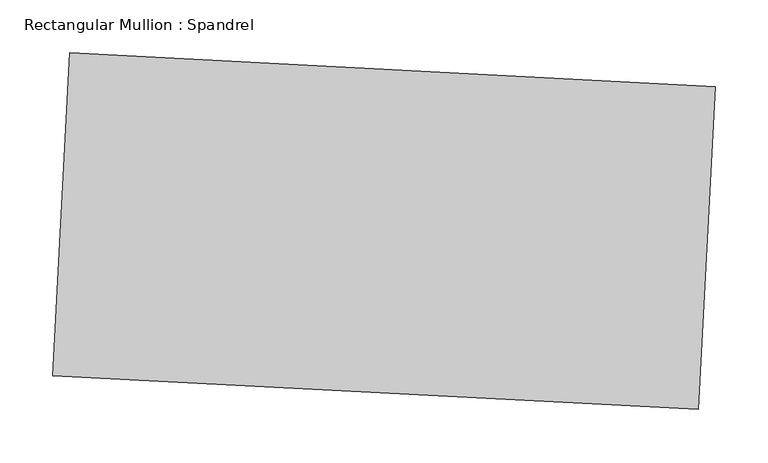
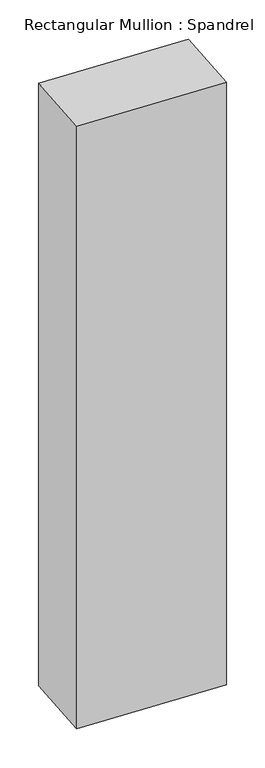
"""IFC4 building model written with IfcOpenShell, lengths in millimetres: member geometry, Rectangular Mullion : Spandrel."""

import ifcopenshell
import ifcopenshell.guid

model = None  # the IFC model being written
_history = None  # IfcOwnerHistory: only IFC2X3 demands one
_inside = {}  # id of a spatial element -> (the spatial element, [elements in it])
_under = {}  # id of a project, library or spatial element -> (it, [spatial elements below it])
_declared = {}  # id of a project -> (the project, [libraries it declares])
_typed = {}  # id of a type object -> (the type object, [elements of that type])
_made_of = {}  # id of a material, layer set ... -> (it, [elements and type objects made of it])


def new_model(schema):
    """Start an empty IFC model of exactly this schema.

    Asked for "IFC4X3", IfcOpenShell would pick the latest addendum, in which some entities
    have other attributes; the version numbers below select the first issue.
    IFC2X3 requires an IfcOwnerHistory on every rooted entity: one is made here for all.
    """
    global model, _history
    if schema == "IFC4X3":
        model = ifcopenshell.file(schema_version=(4, 3, 0, 0))
    else:
        model = ifcopenshell.file(schema=schema)
    _inside.clear()
    _under.clear()
    _declared.clear()
    _typed.clear()
    _made_of.clear()
    _history = None
    if model.schema == "IFC2X3":
        org = make("IfcOrganization", Name="unknown")
        user = make(
            "IfcPersonAndOrganization",
            ThePerson=make("IfcPerson", FamilyName="unknown"),
            TheOrganization=org,
        )
        app = make(
            "IfcApplication",
            ApplicationDeveloper=org,
            Version="unknown",
            ApplicationFullName="unknown",
            ApplicationIdentifier="unknown",
        )
        _history = make(
            "IfcOwnerHistory",
            OwningUser=user,
            OwningApplication=app,
            ChangeAction="ADDED",
            CreationDate=0,
        )
    return model


def make(cls, **values):
    """One entity of the class cls with the attributes given. An attribute that is None is left unset."""
    return model.create_entity(
        cls, **{name: value for name, value in values.items() if value is not None}
    )


def rooted(cls, **values):
    """An entity with a GlobalId (a new one), such as an element, a storey or a relation."""
    return make(cls, GlobalId=ifcopenshell.guid.new(), OwnerHistory=_history, **values)


def si_unit(unit_type, name, prefix=None):
    """IfcSIUnit, for example si_unit("LENGTHUNIT", "METRE", prefix="MILLI")."""
    return make("IfcSIUnit", UnitType=unit_type, Prefix=prefix, Name=name)


def assignment(units):
    """IfcUnitAssignment: the units of a project."""
    return None if units is None else make("IfcUnitAssignment", Units=units)


def point(xyz):
    """IfcCartesianPoint."""
    return None if xyz is None else make("IfcCartesianPoint", Coordinates=xyz)


def direction(xyz):
    """IfcDirection."""
    return None if xyz is None else make("IfcDirection", DirectionRatios=xyz)


def frame(location, z_axis=None, x_axis=None):
    """IfcAxis2Placement3D, a coordinate frame: its origin and axes. An axis left out is left unset."""
    return make(
        "IfcAxis2Placement3D",
        Location=point(location),
        Axis=direction(z_axis),
        RefDirection=direction(x_axis),
    )


def origin():
    """The frame at (0, 0, 0) with its axes left unset."""
    return frame((0.0, 0.0, 0.0))


def place(relative_to, where):
    """IfcLocalPlacement: puts the frame where relative to a parent placement (None: the world)."""
    return make(
        "IfcLocalPlacement", PlacementRelTo=relative_to, RelativePlacement=where
    )


def context(
    kind, dimensions, precision=None, world=None, true_north=None, identifier=None
):
    """IfcGeometricRepresentationContext, for example the 3D "Model" context."""
    return make(
        "IfcGeometricRepresentationContext",
        ContextIdentifier=identifier,
        ContextType=kind,
        CoordinateSpaceDimension=dimensions,
        Precision=precision,
        WorldCoordinateSystem=world,
        TrueNorth=true_north,
    )


def project(units=None, contexts=None):
    """IfcProject with its units and contexts."""
    return rooted(
        "IfcProject",
        Name="project",
        RepresentationContexts=contexts,
        UnitsInContext=assignment(units),
    )


def spatial(cls, under=None, at=None, **own):
    """A site, building, storey or space (cls), placed at a placement, below another one or the project."""
    s = rooted(cls, ObjectPlacement=at, **own)
    if under is not None:
        _under.setdefault(under.id(), (under, []))[1].append(s)
    return s


def polyline(points):
    """IfcPolyline through the points."""
    return make("IfcPolyline", Points=[point(p) for p in points])


def outline(outer, holes=None, kind="AREA"):
    """IfcArbitraryClosedProfileDef: a profile drawn as a closed curve; with holes, ...WithVoids."""
    if holes is None:
        return make("IfcArbitraryClosedProfileDef", ProfileType=kind, OuterCurve=outer)
    return make(
        "IfcArbitraryProfileDefWithVoids",
        ProfileType=kind,
        OuterCurve=outer,
        InnerCurves=holes,
    )


def extrude(swept, where, along, depth):
    """IfcExtrudedAreaSolid: the profile swept, set in the frame where, extruded along a direction by depth."""
    return make(
        "IfcExtrudedAreaSolid",
        SweptArea=swept,
        Position=where,
        ExtrudedDirection=direction(along),
        Depth=depth,
    )


def shape(context_of_items, identifier, shape_type, items):
    """IfcShapeRepresentation: the items that make up one representation, for example the "Body"."""
    return make(
        "IfcShapeRepresentation",
        ContextOfItems=context_of_items,
        RepresentationIdentifier=identifier,
        RepresentationType=shape_type,
        Items=items,
    )


def source(mapping_origin, context_of_items, identifier, shape_type, items):
    """IfcRepresentationMap: a shape defined once, which mapped items show again and again."""
    return make(
        "IfcRepresentationMap",
        MappingOrigin=mapping_origin,
        MappedRepresentation=shape(context_of_items, identifier, shape_type, items),
    )


def transform(
    local_origin,
    x_axis=None,
    y_axis=None,
    z_axis=None,
    scale=None,
    scale2=None,
    scale3=None,
    uniform=True,
):
    """IfcCartesianTransformationOperator3D, or its non-uniform kind. x_axis, y_axis, z_axis: its Axis1, 2, 3."""
    if uniform:
        return make(
            "IfcCartesianTransformationOperator3D",
            Axis1=direction(x_axis),
            Axis2=direction(y_axis),
            LocalOrigin=point(local_origin),
            Scale=scale,
            Axis3=direction(z_axis),
        )
    return make(
        "IfcCartesianTransformationOperator3DnonUniform",
        Axis1=direction(x_axis),
        Axis2=direction(y_axis),
        LocalOrigin=point(local_origin),
        Scale=scale,
        Axis3=direction(z_axis),
        Scale2=scale2,
        Scale3=scale3,
    )


def mapped(mapping_source, mapping_target):
    """IfcMappedItem: shows the shape of a source again, moved by a transform."""
    return make(
        "IfcMappedItem", MappingSource=mapping_source, MappingTarget=mapping_target
    )


def made_of(thing, what):
    """Note that an element or type object is made of a material, layer set ...; save() writes the relation."""
    if what is not None:
        _made_of.setdefault(what.id(), (what, []))[1].append(thing)
    return thing


def element(
    cls,
    number,
    at=None,
    inside=None,
    cuts=None,
    type_object=None,
    material=None,
    context=None,
    identifier="Body",
    shape_type=None,
    held_by="IfcProductDefinitionShape",
    body=None,
    shapes=None,
    **own,
):
    """One element of the class cls, such as IfcWall. Its Tag is "e" and its number.

    at: its placement. inside: the storey or other place that contains it. cuts: it is an
    opening in that element (IfcRelVoidsElement). A single representation is given by context,
    identifier, shape_type and body (its items); several are given by shapes. held_by: the class
    of the entity that holds the representations. save() writes the other relations.
    """
    e = rooted(cls, Tag="e%d" % number, ObjectPlacement=at, **own)
    if body is not None:
        shapes = [shape(context, identifier, shape_type, body)]
    if shapes is not None:
        e.Representation = make(held_by, Representations=shapes)
    if inside is not None:
        _inside.setdefault(inside.id(), (inside, []))[1].append(e)
    if cuts is not None:
        rooted(
            "IfcRelVoidsElement", RelatingBuildingElement=cuts, RelatedOpeningElement=e
        )
    if type_object is not None:
        _typed.setdefault(type_object.id(), (type_object, []))[1].append(e)
    return made_of(e, material)


def aggregate(whole, parts):
    """IfcRelAggregates: a whole, such as a stair, and the parts it consists of."""
    return rooted("IfcRelAggregates", RelatingObject=whole, RelatedObjects=parts)


def save(model, path):
    """Write the relations noted so far, then the file.

    IfcRelAggregates (storeys below a building ...), IfcRelContainedInSpatialStructure (elements
    in a storey), IfcRelDefinesByType, IfcRelAssociatesMaterial and IfcRelDeclares: one each for
    every whole, place, type object, material and project.
    """
    for whole, parts in _under.values():
        aggregate(whole, parts)
    for where, things in _inside.values():
        rooted(
            "IfcRelContainedInSpatialStructure",
            RelatedElements=things,
            RelatingStructure=where,
        )
    for kind, things in _typed.values():
        rooted("IfcRelDefinesByType", RelatedObjects=things, RelatingType=kind)
    for what, things in _made_of.values():
        rooted("IfcRelAssociatesMaterial", RelatedObjects=things, RelatingMaterial=what)
    for by, libraries in _declared.values():
        rooted("IfcRelDeclares", RelatingContext=by, RelatedDefinitions=libraries)
    model.write(path)


def rectangular_mullion_spandrel_2df0ba9b(model_context):
    return source(origin(), model_context, "Body", "SweptSolid", [
        extrude(outline(polyline([(312.3582819, 136.2391416), (296.4062825, -168.1431406), (-312.3582819, -136.2391416), (-296.4062825, 168.1431406), (312.3582819, 136.2391416)])), frame((0.0, 0.0, -2667.6321869), z_axis=(0.0, 0.0, 1.0), x_axis=(1.0, 0.0, 0.0)), (0.0, 0.0, 1.0), 2667.6321869),
    ])


if __name__ == "__main__":
    model = new_model("IFC4")
    model_context = context("Model", 3, world=origin())
    ifc_project = project(units=[si_unit("LENGTHUNIT", "METRE", prefix="MILLI")], contexts=[model_context])
    site = spatial("IfcSite", under=ifc_project)
    building = spatial("IfcBuilding", under=site)
    placement = place(None, origin())
    rectangular_mullion_spandrel_shape = rectangular_mullion_spandrel_2df0ba9b(model_context)
    element("IfcMember", 1, ObjectType="Rectangular Mullion : Spandrel", at=placement, inside=building, context=model_context, shape_type="MappedRepresentation", body=[
        mapped(rectangular_mullion_spandrel_shape, transform((0.0, 0.0, 0.0), x_axis=(1.0, 0.0, 0.0), y_axis=(0.0, 1.0, 0.0), z_axis=(0.0, 0.0, 1.0))),
    ])
    save(model, "model.ifc")

# Revit data of these elements
# Type "Rectangular Mullion : Spandrel"
#   built-in parameter 1007304 = 1 (stored number, unit not read)
#   built-in parameter 1007301 = 1 (stored number, unit not read)
#   built-in parameter 1007300 = 1 (stored number, unit not read)
# Element 1 (IfcMember, "Rectangular Mullion : Spandrel")
#   Materials on its faces: "Aluminum"
# Materials
#   "Aluminum": class "Metal", colour RGB 247 247 247, transparency 0, Description = "Aluminum 6061", Cost = 0
